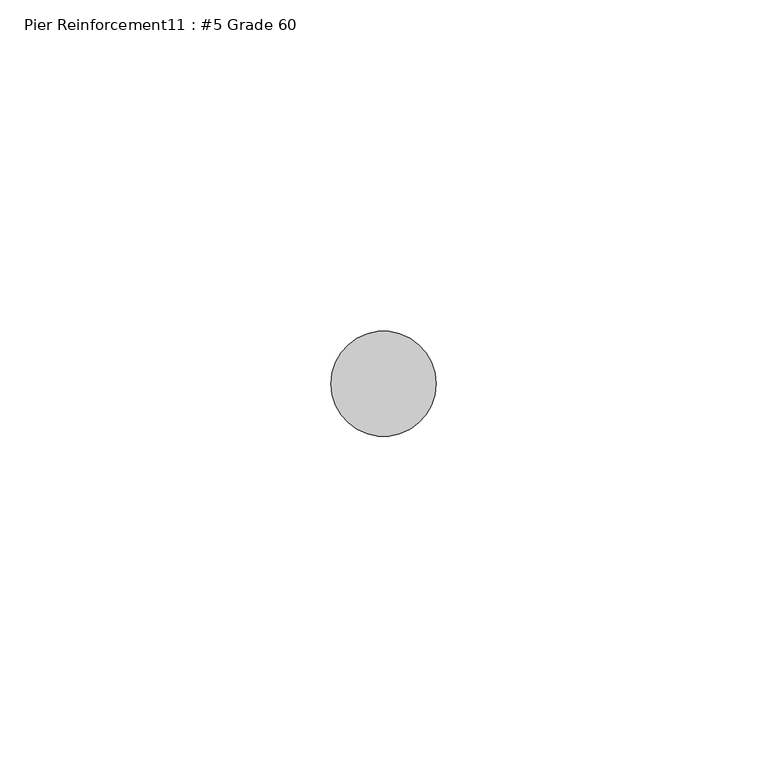
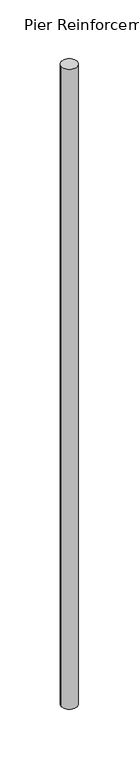
"""IFC4 building model written with IfcOpenShell, lengths in millimetres: proxy geometry, Pier Reinforcement11 : #5 Grade 60."""

import ifcopenshell
import ifcopenshell.guid

model = None  # the IFC model being written
_history = None  # IfcOwnerHistory: only IFC2X3 demands one
_inside = {}  # id of a spatial element -> (the spatial element, [elements in it])
_under = {}  # id of a project, library or spatial element -> (it, [spatial elements below it])
_declared = {}  # id of a project -> (the project, [libraries it declares])
_typed = {}  # id of a type object -> (the type object, [elements of that type])
_made_of = {}  # id of a material, layer set ... -> (it, [elements and type objects made of it])


def new_model(schema):
    """Start an empty IFC model of exactly this schema.

    Asked for "IFC4X3", IfcOpenShell would pick the latest addendum, in which some entities
    have other attributes; the version numbers below select the first issue.
    IFC2X3 requires an IfcOwnerHistory on every rooted entity: one is made here for all.
    """
    global model, _history
    if schema == "IFC4X3":
        model = ifcopenshell.file(schema_version=(4, 3, 0, 0))
    else:
        model = ifcopenshell.file(schema=schema)
    _inside.clear()
    _under.clear()
    _declared.clear()
    _typed.clear()
    _made_of.clear()
    _history = None
    if model.schema == "IFC2X3":
        org = make("IfcOrganization", Name="unknown")
        user = make(
            "IfcPersonAndOrganization",
            ThePerson=make("IfcPerson", FamilyName="unknown"),
            TheOrganization=org,
        )
        app = make(
            "IfcApplication",
            ApplicationDeveloper=org,
            Version="unknown",
            ApplicationFullName="unknown",
            ApplicationIdentifier="unknown",
        )
        _history = make(
            "IfcOwnerHistory",
            OwningUser=user,
            OwningApplication=app,
            ChangeAction="ADDED",
            CreationDate=0,
        )
    return model


def make(cls, **values):
    """One entity of the class cls with the attributes given. An attribute that is None is left unset."""
    return model.create_entity(
        cls, **{name: value for name, value in values.items() if value is not None}
    )


def rooted(cls, **values):
    """An entity with a GlobalId (a new one), such as an element, a storey or a relation."""
    return make(cls, GlobalId=ifcopenshell.guid.new(), OwnerHistory=_history, **values)


def si_unit(unit_type, name, prefix=None):
    """IfcSIUnit, for example si_unit("LENGTHUNIT", "METRE", prefix="MILLI")."""
    return make("IfcSIUnit", UnitType=unit_type, Prefix=prefix, Name=name)


def assignment(units):
    """IfcUnitAssignment: the units of a project."""
    return None if units is None else make("IfcUnitAssignment", Units=units)


def point(xyz):
    """IfcCartesianPoint."""
    return None if xyz is None else make("IfcCartesianPoint", Coordinates=xyz)


def direction(xyz):
    """IfcDirection."""
    return None if xyz is None else make("IfcDirection", DirectionRatios=xyz)


def frame(location, z_axis=None, x_axis=None):
    """IfcAxis2Placement3D, a coordinate frame: its origin and axes. An axis left out is left unset."""
    return make(
        "IfcAxis2Placement3D",
        Location=point(location),
        Axis=direction(z_axis),
        RefDirection=direction(x_axis),
    )


def frame_2d(location, x_axis=None):
    """IfcAxis2Placement2D, a coordinate frame in the plane: its origin and x axis."""
    return make(
        "IfcAxis2Placement2D", Location=point(location), RefDirection=direction(x_axis)
    )


def origin():
    """The frame at (0, 0, 0) with its axes left unset."""
    return frame((0.0, 0.0, 0.0))


def place(relative_to, where):
    """IfcLocalPlacement: puts the frame where relative to a parent placement (None: the world)."""
    return make(
        "IfcLocalPlacement", PlacementRelTo=relative_to, RelativePlacement=where
    )


def context(
    kind, dimensions, precision=None, world=None, true_north=None, identifier=None
):
    """IfcGeometricRepresentationContext, for example the 3D "Model" context."""
    return make(
        "IfcGeometricRepresentationContext",
        ContextIdentifier=identifier,
        ContextType=kind,
        CoordinateSpaceDimension=dimensions,
        Precision=precision,
        WorldCoordinateSystem=world,
        TrueNorth=true_north,
    )


def project(units=None, contexts=None):
    """IfcProject with its units and contexts."""
    return rooted(
        "IfcProject",
        Name="project",
        RepresentationContexts=contexts,
        UnitsInContext=assignment(units),
    )


def spatial(cls, under=None, at=None, **own):
    """A site, building, storey or space (cls), placed at a placement, below another one or the project."""
    s = rooted(cls, ObjectPlacement=at, **own)
    if under is not None:
        _under.setdefault(under.id(), (under, []))[1].append(s)
    return s


def circle_curve(where, radius):
    """IfcCircle in the frame where."""
    return make("IfcCircle", Position=where, Radius=radius)


def trimmed(basis, trim1, trim2, sense, master):
    """IfcTrimmedCurve: the piece of a basis curve between two trims."""
    return make(
        "IfcTrimmedCurve",
        BasisCurve=basis,
        Trim1=trim1,
        Trim2=trim2,
        SenseAgreement=sense,
        MasterRepresentation=master,
    )


def segment(curve, same_sense, transition):
    """IfcCompositeCurveSegment."""
    return make(
        "IfcCompositeCurveSegment",
        Transition=transition,
        SameSense=same_sense,
        ParentCurve=curve,
    )


def composite_curve(segments, self_intersect=None):
    """IfcCompositeCurve: segments joined end to end."""
    return make("IfcCompositeCurve", Segments=segments, SelfIntersect=self_intersect)


def outline(outer, holes=None, kind="AREA"):
    """IfcArbitraryClosedProfileDef: a profile drawn as a closed curve; with holes, ...WithVoids."""
    if holes is None:
        return make("IfcArbitraryClosedProfileDef", ProfileType=kind, OuterCurve=outer)
    return make(
        "IfcArbitraryProfileDefWithVoids",
        ProfileType=kind,
        OuterCurve=outer,
        InnerCurves=holes,
    )


def extrude(swept, where, along, depth):
    """IfcExtrudedAreaSolid: the profile swept, set in the frame where, extruded along a direction by depth."""
    return make(
        "IfcExtrudedAreaSolid",
        SweptArea=swept,
        Position=where,
        ExtrudedDirection=direction(along),
        Depth=depth,
    )


def shape(context_of_items, identifier, shape_type, items):
    """IfcShapeRepresentation: the items that make up one representation, for example the "Body"."""
    return make(
        "IfcShapeRepresentation",
        ContextOfItems=context_of_items,
        RepresentationIdentifier=identifier,
        RepresentationType=shape_type,
        Items=items,
    )


def source(mapping_origin, context_of_items, identifier, shape_type, items):
    """IfcRepresentationMap: a shape defined once, which mapped items show again and again."""
    return make(
        "IfcRepresentationMap",
        MappingOrigin=mapping_origin,
        MappedRepresentation=shape(context_of_items, identifier, shape_type, items),
    )


def transform(
    local_origin,
    x_axis=None,
    y_axis=None,
    z_axis=None,
    scale=None,
    scale2=None,
    scale3=None,
    uniform=True,
):
    """IfcCartesianTransformationOperator3D, or its non-uniform kind. x_axis, y_axis, z_axis: its Axis1, 2, 3."""
    if uniform:
        return make(
            "IfcCartesianTransformationOperator3D",
            Axis1=direction(x_axis),
            Axis2=direction(y_axis),
            LocalOrigin=point(local_origin),
            Scale=scale,
            Axis3=direction(z_axis),
        )
    return make(
        "IfcCartesianTransformationOperator3DnonUniform",
        Axis1=direction(x_axis),
        Axis2=direction(y_axis),
        LocalOrigin=point(local_origin),
        Scale=scale,
        Axis3=direction(z_axis),
        Scale2=scale2,
        Scale3=scale3,
    )


def mapped(mapping_source, mapping_target):
    """IfcMappedItem: shows the shape of a source again, moved by a transform."""
    return make(
        "IfcMappedItem", MappingSource=mapping_source, MappingTarget=mapping_target
    )


def made_of(thing, what):
    """Note that an element or type object is made of a material, layer set ...; save() writes the relation."""
    if what is not None:
        _made_of.setdefault(what.id(), (what, []))[1].append(thing)
    return thing


def element(
    cls,
    number,
    at=None,
    inside=None,
    cuts=None,
    type_object=None,
    material=None,
    context=None,
    identifier="Body",
    shape_type=None,
    held_by="IfcProductDefinitionShape",
    body=None,
    shapes=None,
    **own,
):
    """One element of the class cls, such as IfcWall. Its Tag is "e" and its number.

    at: its placement. inside: the storey or other place that contains it. cuts: it is an
    opening in that element (IfcRelVoidsElement). A single representation is given by context,
    identifier, shape_type and body (its items); several are given by shapes. held_by: the class
    of the entity that holds the representations. save() writes the other relations.
    """
    e = rooted(cls, Tag="e%d" % number, ObjectPlacement=at, **own)
    if body is not None:
        shapes = [shape(context, identifier, shape_type, body)]
    if shapes is not None:
        e.Representation = make(held_by, Representations=shapes)
    if inside is not None:
        _inside.setdefault(inside.id(), (inside, []))[1].append(e)
    if cuts is not None:
        rooted(
            "IfcRelVoidsElement", RelatingBuildingElement=cuts, RelatedOpeningElement=e
        )
    if type_object is not None:
        _typed.setdefault(type_object.id(), (type_object, []))[1].append(e)
    return made_of(e, material)


def aggregate(whole, parts):
    """IfcRelAggregates: a whole, such as a stair, and the parts it consists of."""
    return rooted("IfcRelAggregates", RelatingObject=whole, RelatedObjects=parts)


def save(model, path):
    """Write the relations noted so far, then the file.

    IfcRelAggregates (storeys below a building ...), IfcRelContainedInSpatialStructure (elements
    in a storey), IfcRelDefinesByType, IfcRelAssociatesMaterial and IfcRelDeclares: one each for
    every whole, place, type object, material and project.
    """
    for whole, parts in _under.values():
        aggregate(whole, parts)
    for where, things in _inside.values():
        rooted(
            "IfcRelContainedInSpatialStructure",
            RelatedElements=things,
            RelatingStructure=where,
        )
    for kind, things in _typed.values():
        rooted("IfcRelDefinesByType", RelatedObjects=things, RelatingType=kind)
    for what, things in _made_of.values():
        rooted("IfcRelAssociatesMaterial", RelatedObjects=things, RelatingMaterial=what)
    for by, libraries in _declared.values():
        rooted("IfcRelDeclares", RelatingContext=by, RelatedDefinitions=libraries)
    model.write(path)


def pier_reinforcement11_5_grade_60_3acffefc(model_context):
    return source(origin(), model_context, "Body", "SweptSolid", [
        extrude(outline(composite_curve([segment(trimmed(circle_curve(frame_2d((590226.0547365, -534096.6663841)), 7.9375), [point((590218.1172365, -534096.6663841))], [point((590233.9922365, -534096.6663841))], False, "CARTESIAN"), True, "CONTINUOUS"), segment(trimmed(circle_curve(frame_2d((590226.0547365, -534096.6663841)), 7.9375), [point((590233.9922365, -534096.6663841))], [point((590218.1172365, -534096.6663841))], False, "CARTESIAN"), True, "CONTINUOUS")], self_intersect=False)), frame((0.0, 0.0, -733.425), z_axis=(0.0, 0.0, 1.0), x_axis=(1.0, 0.0, 0.0)), (0.0, 0.0, 1.0), 685.8),
    ])


if __name__ == "__main__":
    model = new_model("IFC4")
    model_context = context("Model", 3, world=origin())
    ifc_project = project(units=[si_unit("LENGTHUNIT", "METRE", prefix="MILLI")], contexts=[model_context])
    site = spatial("IfcSite", under=ifc_project)
    building = spatial("IfcBuilding", under=site)
    placement = place(None, origin())
    pier_reinforcement11_5_grade_60_shape = pier_reinforcement11_5_grade_60_3acffefc(model_context)
    element("IfcBuildingElementProxy", 1, Name="Pier Reinforcement11 : #5 Grade 60", ObjectType="Pier Reinforcement11 : #5 Grade 60", at=placement, inside=building, context=model_context, shape_type="MappedRepresentation", body=[
        mapped(pier_reinforcement11_5_grade_60_shape, transform((0.0, 0.0, 0.0), x_axis=(1.0, 0.0, 0.0), y_axis=(0.0, 1.0, 0.0), z_axis=(0.0, 0.0, 1.0))),
    ])
    save(model, "model.ifc")

# Revit data of these elements
# Element 1 (IfcBuildingElementProxy, "Pier Reinforcement11 : #5 Grade 60")
#   Materials on its faces: "#4 GR. 60 REINF. @ 16\" O.C. EW."
# Materials
#   "#4 GR. 60 REINF. @ 16\" O.C. EW.": class "Generic", colour RGB 84 83 81, transparency 0, Cost = 0
